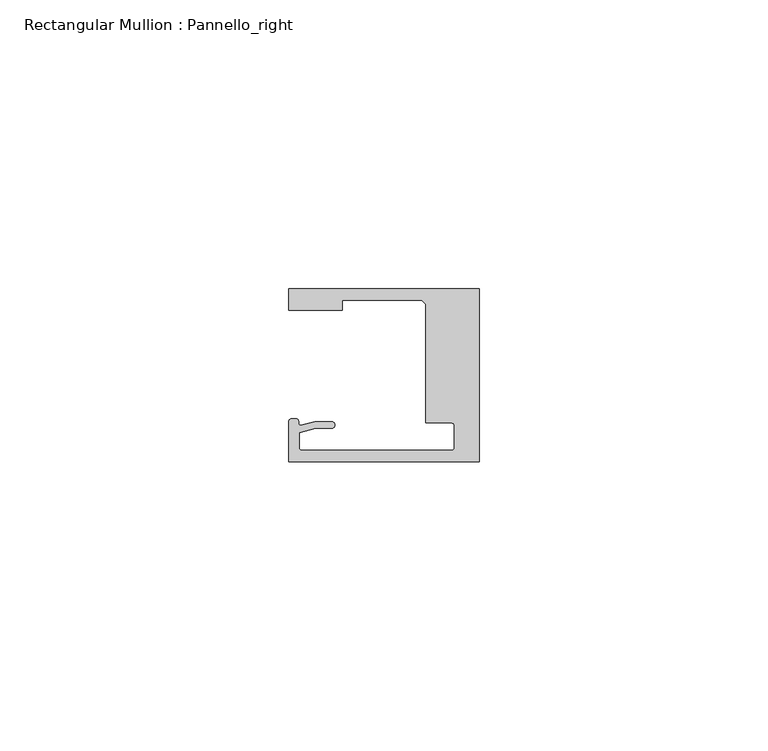
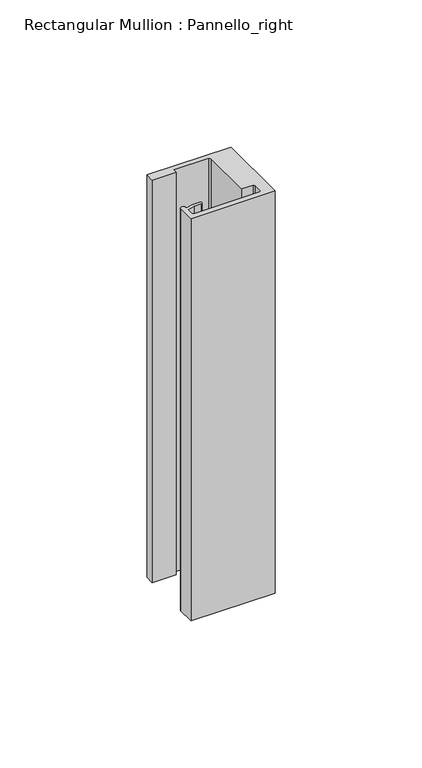
"""IFC4 building model written with IfcOpenShell, lengths in millimetres: member geometry, Rectangular Mullion : Pannello_right."""

from ifc_helpers import new_model, si_unit, frame, origin, place, context, project, spatial, polyline, circle_curve, source, transform, mapped, element, save
from ifc_brep_helpers import plane_surface, cylinder_surface, revolved_surface, extruded_surface, spline_curve, advanced_brep


def rectangular_mullion_pannello_right_cbba8e2e(model_context):
    return source(origin(), model_context, "Body", "AdvancedBrep", [
        advanced_brep(
        [(-33.0, 15.0, 0.0), (-33.0, 11.3000004, 0.0), (-23.700041, 11.3000004, 0.0), (-23.700041, 13.0000004, 0.0), (-10.0000103, 13.0000004, 0.0), (-9.2999726, 12.2999849, 0.0), (-9.2999726, -8.2500595, 0.0), (-4.7999726, -8.2500595, 0.0), (-4.2999726, -8.7500595, 0.0), (-4.2999726, -12.50001, 0.0), (-4.7999726, -13.00001, 0.0), (-30.69998, -13.00001, 0.0), (-31.19998, -12.50001, 0.0), (-31.19998, -9.9657591, 0.0), (-28.3419477, -9.1999523, 0.0), (-25.59998, -9.1999523, 0.0), (-25.59998, -7.9999523, 0.0), (-28.4999305, -7.9999523, 0.0), (-30.9223017, -8.6490241, 0.0), (-33.0000135, -8.0000472, 0.0), (-33.0000135, -15.0, 0.0), (0.0, -15.0, 0.0), (0.0, 15.0, 0.0), (-33.0, 15.0, -166.9999865), (0.0, 15.0, -166.9999865), (0.0, -15.0, -166.9999865), (-33.0000135, -15.0, -166.9999865), (-33.0000135, -8.0000472, -166.9999865), (-30.9223017, -8.6490241, -166.9999865), (-28.4999305, -7.9999523, -166.9999865), (-25.59998, -7.9999523, -166.9999865), (-25.59998, -9.1999523, -166.9999865), (-28.3419477, -9.1999523, -166.9999865), (-31.19998, -9.9657591, -166.9999865), (-31.19998, -12.50001, -166.9999865), (-30.69998, -13.00001, -166.9999865), (-4.7999726, -13.00001, -166.9999865), (-4.2999726, -12.50001, -166.9999865), (-4.2999726, -8.7500595, -166.9999865), (-4.7999726, -8.2500595, -166.9999865), (-9.2999726, -8.2500595, -166.9999865), (-9.2999726, 12.2999849, -166.9999865), (-10.0000103, 13.0000004, -166.9999865), (-23.700041, 13.0000004, -166.9999865), (-23.700041, 11.3000004, -166.9999865), (-33.0, 11.3000004, -166.9999865)],
        [
            (0, 1),
            (1, 2),
            (2, 3),
            (3, 4),
            (4, 5),
            (5, 6),
            (6, 7),
            (7, 8, circle_curve(frame((-4.7999726, -8.7500595, 0.0), z_axis=(0.0, 0.0, -1.0), x_axis=(0.0, 1.0, 0.0)), 0.5)),
            (8, 9),
            (9, 10, circle_curve(frame((-4.7999726, -12.50001, 0.0), z_axis=(0.0, 0.0, -1.0), x_axis=(1.0, 0.0, 0.0)), 0.5)),
            (10, 11),
            (11, 12, circle_curve(frame((-30.69998, -12.50001, 0.0), z_axis=(0.0, 0.0, -1.0), x_axis=(0.0, -1.0, 0.0)), 0.5)),
            (12, 13),
            (13, 14),
            (14, 15),
            (15, 16, circle_curve(frame((-25.59998, -8.5999523, 0.0), z_axis=(0.0, 0.0, 1.0), x_axis=(0.0, -1.0, 0.0)), 0.6)),
            (16, 17),
            (17, 18),
            (18, 19, spline_curve(3, [(-30.9223017, -8.6490241, 0.0), (-31.312054066, -8.717747958, 0.0), (-31.298563602, -8.366228555, 0.0), (-31.305645054, -7.690065204, 0.0), (-31.357433266, -7.563996614, 0.0), (-32.262327879, -7.456527435, 0.0), (-33.0000135, -7.457047519, 0.0), (-33.0000135, -8.0000472, 0.0)], [4, 2, 2, 4], [0.0, 0.001840817752199412, 0.004996616814974408, 0.007702013405570312])),
            (19, 20),
            (20, 21),
            (21, 22),
            (22, 0),
            (23, 24),
            (24, 25),
            (25, 26),
            (26, 27),
            (27, 28, spline_curve(3, [(-33.0000135, -8.0000472, -166.9999865), (-33.0000135, -7.457047519, -166.9999865), (-32.262327879, -7.456527435, -166.9999865), (-31.357433266, -7.563996614, -166.9999865), (-31.305645054, -7.690065204, -166.9999865), (-31.298563602, -8.366228555, -166.9999865), (-31.312054066, -8.717747958, -166.9999865), (-30.9223017, -8.6490241, -166.9999865)], [4, 2, 2, 4], [0.0, 0.0027053965905959043, 0.0058611956533709, 0.007702013405570312])),
            (28, 29),
            (29, 30),
            (30, 31, circle_curve(frame((-25.59998, -8.5999523, -166.9999865), z_axis=(0.0, 0.0, -1.0), x_axis=(0.0, -1.0, 0.0)), 0.6)),
            (31, 32),
            (32, 33),
            (33, 34),
            (34, 35, circle_curve(frame((-30.69998, -12.50001, -166.9999865), z_axis=(0.0, 0.0, 1.0), x_axis=(0.0, -1.0, 0.0)), 0.5)),
            (35, 36),
            (36, 37, circle_curve(frame((-4.7999726, -12.50001, -166.9999865), z_axis=(0.0, 0.0, 1.0), x_axis=(1.0, 0.0, 0.0)), 0.5)),
            (37, 38),
            (38, 39, circle_curve(frame((-4.7999726, -8.7500595, -166.9999865), z_axis=(0.0, 0.0, 1.0), x_axis=(0.0, 1.0, 0.0)), 0.5)),
            (39, 40),
            (40, 41),
            (41, 42),
            (42, 43),
            (43, 44),
            (44, 45),
            (45, 23),
            (0, 23),
            (45, 1),
            (44, 2),
            (43, 3),
            (42, 4),
            (41, 5),
            (40, 6),
            (39, 7),
            (38, 8),
            (37, 9),
            (36, 10),
            (35, 11),
            (34, 12),
            (33, 13),
            (32, 14),
            (31, 15),
            (30, 16),
            (29, 17),
            (28, 18),
            (27, 19),
            (26, 20),
            (25, 21),
            (24, 22),
        ],
        [
            plane_surface(frame((0.0, -36.2491502, 0.0), z_axis=(0.0, 0.0, 1.0), x_axis=(-1.0, 0.0, 0.0))),
            plane_surface(frame((0.0, -36.2491502, -166.9999865), z_axis=(0.0, 0.0, -1.0), x_axis=(-1.0, 0.0, 0.0))),
            plane_surface(frame((-33.0, 15.0, 0.0), z_axis=(-1.0, 0.0, 0.0), x_axis=(0.0, 0.0, -1.0))),
            plane_surface(frame((-33.0, 11.3000004, 0.0), z_axis=(0.0, -1.0, 0.0), x_axis=(0.0, 0.0, -1.0))),
            plane_surface(frame((-23.700041, 11.3000004, 0.0), z_axis=(1.0, 0.0, 0.0), x_axis=(0.0, 0.0, -1.0))),
            plane_surface(frame((-23.700041, 13.0000004, 0.0), z_axis=(0.0, -1.0, 0.0), x_axis=(0.0, 0.0, -1.0))),
            plane_surface(frame((-10.0000103, 13.0000004, 0.0), z_axis=(-0.7070955486278075, -0.7071180135668587, 0.0), x_axis=(0.0, 0.0, -1.0))),
            plane_surface(frame((-9.2999726, 12.2999849, 0.0), z_axis=(-1.0, 0.0, 0.0), x_axis=(0.0, 0.0, -1.0))),
            plane_surface(frame((-9.2999726, -8.2500595, 0.0), z_axis=(0.0, -1.0, 0.0), x_axis=(0.0, 0.0, -1.0))),
            revolved_surface(polyline([(-4.7999726, -8.2500595, -166.9999865), (-4.7999726, -8.2500595, 0.0)]), (-4.7999726, -8.7500595, 0.0), (0.0, 0.0, -1.0)),
            plane_surface(frame((-4.2999726, -8.7500595, 0.0), z_axis=(-1.0, 0.0, 0.0), x_axis=(0.0, 0.0, -1.0))),
            revolved_surface(polyline([(-4.2999726, -12.50001, -166.9999865), (-4.2999726, -12.50001, 0.0)]), (-4.7999726, -12.50001, 0.0), (0.0, 0.0, -1.0)),
            plane_surface(frame((-4.7999726, -13.00001, 0.0), z_axis=(0.0, 1.0, 0.0), x_axis=(0.0, 0.0, -1.0))),
            revolved_surface(polyline([(-30.69998, -13.00001, -166.9999865), (-30.69998, -13.00001, 0.0)]), (-30.69998, -12.50001, 0.0), (0.0, 0.0, -1.0)),
            plane_surface(frame((-31.19998, -12.50001, 0.0), z_axis=(1.0, 0.0, 0.0), x_axis=(0.0, 0.0, -1.0))),
            plane_surface(frame((-31.19998, -9.9657591, 0.0), z_axis=(0.2588188320428738, -0.9659258833782035, 0.0), x_axis=(0.0, 0.0, -1.0))),
            plane_surface(frame((-28.3419477, -9.1999523, 0.0), z_axis=(0.0, -1.0, 0.0), x_axis=(0.0, 0.0, -1.0))),
            cylinder_surface(frame((-25.59998, -8.5999523, 0.0), z_axis=(0.0, 0.0, 1.0), x_axis=(0.0, -1.0, 0.0)), 0.6),
            plane_surface(frame((-25.59998, -7.9999523, 0.0), z_axis=(0.0, 1.0, 0.0), x_axis=(0.0, 0.0, -1.0))),
            plane_surface(frame((-28.4999305, -7.9999523, 0.0), z_axis=(-0.2588188320019168, 0.965925883389178, 0.0), x_axis=(0.0, 0.0, -1.0))),
            extruded_surface(spline_curve(3, [(-30.9223017, -8.6490241, -166.9999865), (-31.312054066, -8.717747958, -166.9999865), (-31.298563602, -8.366228555, -166.9999865), (-31.305645054, -7.690065204, -166.9999865), (-31.357433266, -7.563996614, -166.9999865), (-32.262327879, -7.456527435, -166.9999865), (-33.0000135, -7.457047519, -166.9999865), (-33.0000135, -8.0000472, -166.9999865)], [4, 2, 2, 4], [0.0, 0.001840817752199412, 0.004996616814974408, 0.007702013405570312]), (0.0, 0.0, 166.9999865), 166.9999865),
            plane_surface(frame((-33.0000135, -8.0000472, 0.0), z_axis=(-1.0, 0.0, 0.0), x_axis=(0.0, 0.0, -1.0))),
            plane_surface(frame((-33.0000135, -15.0, 0.0), z_axis=(0.0, -1.0, 0.0), x_axis=(0.0, 0.0, -1.0))),
            plane_surface(frame((0.0, -15.0, 0.0), z_axis=(1.0, 0.0, 0.0), x_axis=(0.0, 0.0, -1.0))),
            plane_surface(frame((0.0, 15.0, 0.0), z_axis=(0.0, 1.0, 0.0), x_axis=(0.0, 0.0, -1.0))),
        ],
        [
            (0, [[1, 2, 3, 4, 5, 6, 7, 8, 9, 10, 11, 12, 13, 14, 15, 16, 17, 18, 19, 20, 21, 22, 23]]),
            (1, [[24, 25, 26, 27, 28, 29, 30, 31, 32, 33, 34, 35, 36, 37, 38, 39, 40, 41, 42, 43, 44, 45, 46]]),
            (2, [[-1, 47, -46, 48]]),
            (3, [[-2, -48, -45, 49]]),
            (4, [[-3, -49, -44, 50]]),
            (5, [[-4, -50, -43, 51]]),
            (6, [[-5, -51, -42, 52]]),
            (7, [[-6, -52, -41, 53]]),
            (8, [[-7, -53, -40, 54]]),
            (9, [[-8, -54, -39, 55]]),
            (10, [[-9, -55, -38, 56]]),
            (11, [[-10, -56, -37, 57]]),
            (12, [[-11, -57, -36, 58]]),
            (13, [[-12, -58, -35, 59]]),
            (14, [[-13, -59, -34, 60]]),
            (15, [[-14, -60, -33, 61]]),
            (16, [[-15, -61, -32, 62]]),
            (17, [[-16, -62, -31, 63]]),
            (18, [[-17, -63, -30, 64]]),
            (19, [[-18, -64, -29, 65]]),
            (20, [[-19, -65, -28, 66]]),
            (21, [[-20, -66, -27, 67]]),
            (22, [[-21, -67, -26, 68]]),
            (23, [[-22, -68, -25, 69]]),
            (24, [[-23, -69, -24, -47]]),
        ],
    ),
    ])


if __name__ == "__main__":
    model = new_model("IFC4")
    model_context = context("Model", 3, world=origin())
    ifc_project = project(units=[si_unit("LENGTHUNIT", "METRE", prefix="MILLI")], contexts=[model_context])
    site = spatial("IfcSite", under=ifc_project)
    building = spatial("IfcBuilding", under=site)
    placement = place(None, origin())
    rectangular_mullion_pannello_right_shape = rectangular_mullion_pannello_right_cbba8e2e(model_context)
    element("IfcMember", 1, ObjectType="Rectangular Mullion : Pannello_right", at=placement, inside=building, context=model_context, shape_type="MappedRepresentation", body=[
        mapped(rectangular_mullion_pannello_right_shape, transform((0.0, 0.0, 0.0), x_axis=(1.0, 0.0, 0.0), y_axis=(0.0, 1.0, 0.0), z_axis=(0.0, 0.0, 1.0))),
    ])
    save(model, "model.ifc")

# Revit data of these elements
# Type "Rectangular Mullion : Pannello_right"
#   built-in parameter 1007322 = 0.0984252 (stored number, unit not read)
#   built-in parameter 1007321 = 0.0305117 (stored number, unit not read)
#   built-in parameter 1007320 = 0 (stored number, unit not read)
